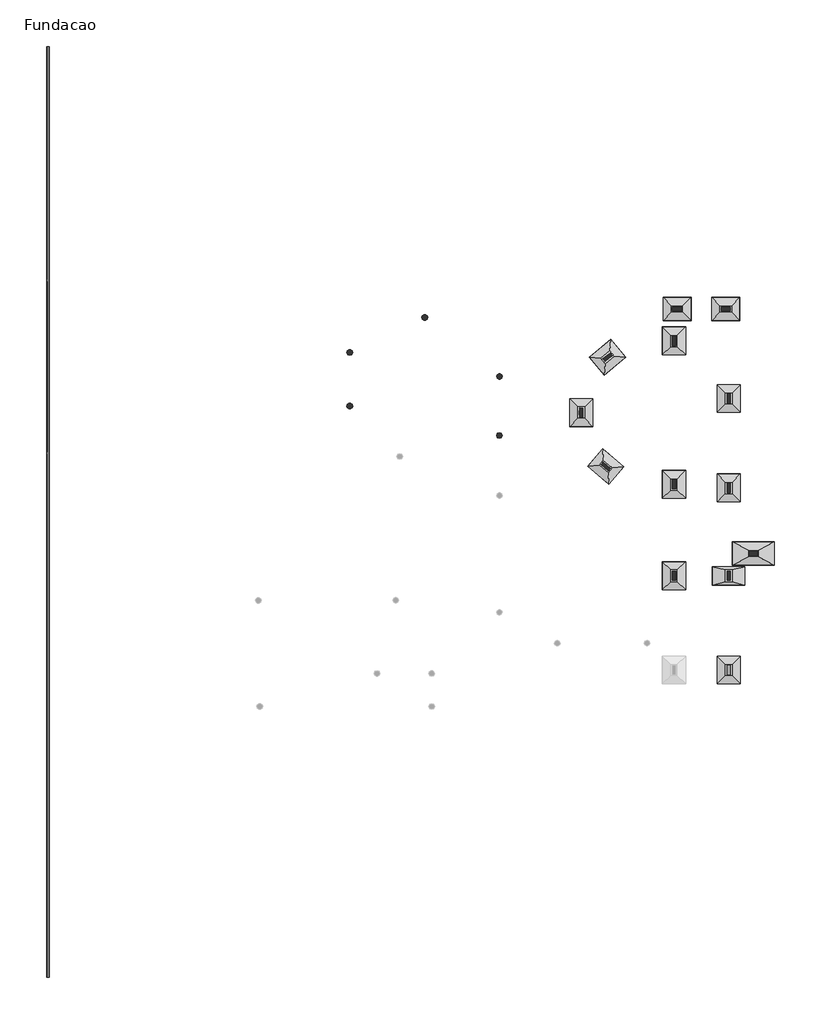
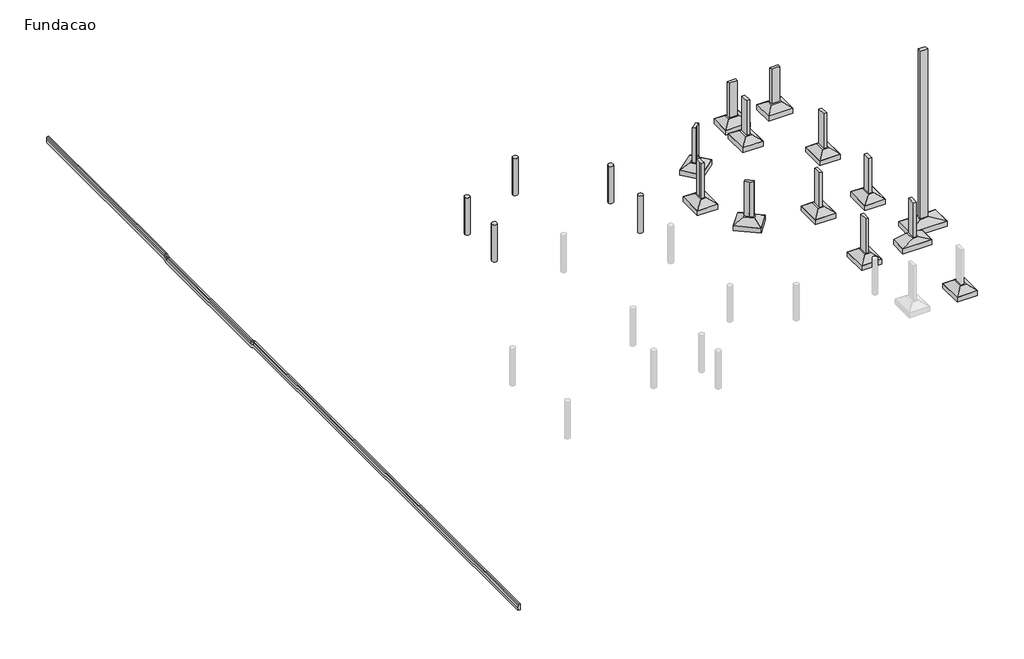
# One storey, part 2 of 2: 17 columns, 13 fasteners, 1 proxy.
"""IFC4 building model written with IfcOpenShell, lengths in millimetres."""

import ifcopenshell
import ifcopenshell.guid

model = None  # the IFC model being written
_history = None  # IfcOwnerHistory: only IFC2X3 demands one
_inside = {}  # id of a spatial element -> (the spatial element, [elements in it])
_under = {}  # id of a project, library or spatial element -> (it, [spatial elements below it])
_declared = {}  # id of a project -> (the project, [libraries it declares])
_typed = {}  # id of a type object -> (the type object, [elements of that type])
_made_of = {}  # id of a material, layer set ... -> (it, [elements and type objects made of it])


def new_model(schema):
    """Start an empty IFC model of exactly this schema.

    Asked for "IFC4X3", IfcOpenShell would pick the latest addendum, in which some entities
    have other attributes; the version numbers below select the first issue.
    IFC2X3 requires an IfcOwnerHistory on every rooted entity: one is made here for all.
    """
    global model, _history
    if schema == "IFC4X3":
        model = ifcopenshell.file(schema_version=(4, 3, 0, 0))
    else:
        model = ifcopenshell.file(schema=schema)
    _inside.clear()
    _under.clear()
    _declared.clear()
    _typed.clear()
    _made_of.clear()
    _history = None
    if model.schema == "IFC2X3":
        org = make("IfcOrganization", Name="unknown")
        user = make(
            "IfcPersonAndOrganization",
            ThePerson=make("IfcPerson", FamilyName="unknown"),
            TheOrganization=org,
        )
        app = make(
            "IfcApplication",
            ApplicationDeveloper=org,
            Version="unknown",
            ApplicationFullName="unknown",
            ApplicationIdentifier="unknown",
        )
        _history = make(
            "IfcOwnerHistory",
            OwningUser=user,
            OwningApplication=app,
            ChangeAction="ADDED",
            CreationDate=0,
        )
    return model


def make(cls, **values):
    """One entity of the class cls with the attributes given. An attribute that is None is left unset."""
    return model.create_entity(
        cls, **{name: value for name, value in values.items() if value is not None}
    )


def rooted(cls, **values):
    """An entity with a GlobalId (a new one), such as an element, a storey or a relation."""
    return make(cls, GlobalId=ifcopenshell.guid.new(), OwnerHistory=_history, **values)


def si_unit(unit_type, name, prefix=None):
    """IfcSIUnit, for example si_unit("LENGTHUNIT", "METRE", prefix="MILLI")."""
    return make("IfcSIUnit", UnitType=unit_type, Prefix=prefix, Name=name)


def assignment(units):
    """IfcUnitAssignment: the units of a project."""
    return None if units is None else make("IfcUnitAssignment", Units=units)


def point(xyz):
    """IfcCartesianPoint."""
    return None if xyz is None else make("IfcCartesianPoint", Coordinates=xyz)


def direction(xyz):
    """IfcDirection."""
    return None if xyz is None else make("IfcDirection", DirectionRatios=xyz)


def frame(location, z_axis=None, x_axis=None):
    """IfcAxis2Placement3D, a coordinate frame: its origin and axes. An axis left out is left unset."""
    return make(
        "IfcAxis2Placement3D",
        Location=point(location),
        Axis=direction(z_axis),
        RefDirection=direction(x_axis),
    )


def origin():
    """The frame at (0, 0, 0) with its axes left unset."""
    return frame((0.0, 0.0, 0.0))


def place(relative_to, where):
    """IfcLocalPlacement: puts the frame where relative to a parent placement (None: the world)."""
    return make(
        "IfcLocalPlacement", PlacementRelTo=relative_to, RelativePlacement=where
    )


def context(
    kind, dimensions, precision=None, world=None, true_north=None, identifier=None
):
    """IfcGeometricRepresentationContext, for example the 3D "Model" context."""
    return make(
        "IfcGeometricRepresentationContext",
        ContextIdentifier=identifier,
        ContextType=kind,
        CoordinateSpaceDimension=dimensions,
        Precision=precision,
        WorldCoordinateSystem=world,
        TrueNorth=true_north,
    )


def project(units=None, contexts=None):
    """IfcProject with its units and contexts."""
    return rooted(
        "IfcProject",
        Name="project",
        RepresentationContexts=contexts,
        UnitsInContext=assignment(units),
    )


def spatial(cls, under=None, at=None, **own):
    """A site, building, storey or space (cls), placed at a placement, below another one or the project."""
    s = rooted(cls, ObjectPlacement=at, **own)
    if under is not None:
        _under.setdefault(under.id(), (under, []))[1].append(s)
    return s


def polyline(points):
    """IfcPolyline through the points."""
    return make("IfcPolyline", Points=[point(p) for p in points])


def circle_curve(where, radius):
    """IfcCircle in the frame where."""
    return make("IfcCircle", Position=where, Radius=radius)


def ellipse_curve(where, semi_axis1, semi_axis2):
    """IfcEllipse in the frame where."""
    return make(
        "IfcEllipse", Position=where, SemiAxis1=semi_axis1, SemiAxis2=semi_axis2
    )


def outline(outer, holes=None, kind="AREA"):
    """IfcArbitraryClosedProfileDef: a profile drawn as a closed curve; with holes, ...WithVoids."""
    if holes is None:
        return make("IfcArbitraryClosedProfileDef", ProfileType=kind, OuterCurve=outer)
    return make(
        "IfcArbitraryProfileDefWithVoids",
        ProfileType=kind,
        OuterCurve=outer,
        InnerCurves=holes,
    )


def extrude(swept, where, along, depth):
    """IfcExtrudedAreaSolid: the profile swept, set in the frame where, extruded along a direction by depth."""
    return make(
        "IfcExtrudedAreaSolid",
        SweptArea=swept,
        Position=where,
        ExtrudedDirection=direction(along),
        Depth=depth,
    )


def faces_of(points, faces, orient=None, outer=None):
    """IfcFace entities. A face is a list of loops; a loop is a list of indices into points, from 0.

    orient and outer hold one flag for each loop. By default every Orientation is true, the
    first loop of a face is its IfcFaceOuterBound and the others are IfcFaceBound.
    """
    made = []
    for i, loops in enumerate(faces):
        bounds = []
        for j, loop in enumerate(loops):
            is_outer = j == 0 if outer is None else outer[i][j]
            bounds.append(
                make(
                    "IfcFaceOuterBound" if is_outer else "IfcFaceBound",
                    Bound=make("IfcPolyLoop", Polygon=[points[k] for k in loop]),
                    Orientation=True if orient is None else orient[i][j],
                )
            )
        made.append(make("IfcFace", Bounds=bounds))
    return made


def faceted_brep(points, faces, orient=None, outer=None, voids=None):
    """IfcFacetedBrep: a solid bounded by flat faces; with voids (closed shells), ...WithVoids."""
    shared = [point(p) for p in points]
    hull = make("IfcClosedShell", CfsFaces=faces_of(shared, faces, orient, outer))
    if voids is None:
        return make("IfcFacetedBrep", Outer=hull)
    return make(
        "IfcFacetedBrepWithVoids",
        Outer=hull,
        Voids=[
            make(cls, CfsFaces=faces_of(shared, fs, o, b)) for cls, fs, o, b in voids
        ],
    )


def shape(context_of_items, identifier, shape_type, items):
    """IfcShapeRepresentation: the items that make up one representation, for example the "Body"."""
    return make(
        "IfcShapeRepresentation",
        ContextOfItems=context_of_items,
        RepresentationIdentifier=identifier,
        RepresentationType=shape_type,
        Items=items,
    )


def source(mapping_origin, context_of_items, identifier, shape_type, items):
    """IfcRepresentationMap: a shape defined once, which mapped items show again and again."""
    return make(
        "IfcRepresentationMap",
        MappingOrigin=mapping_origin,
        MappedRepresentation=shape(context_of_items, identifier, shape_type, items),
    )


def transform(
    local_origin,
    x_axis=None,
    y_axis=None,
    z_axis=None,
    scale=None,
    scale2=None,
    scale3=None,
    uniform=True,
):
    """IfcCartesianTransformationOperator3D, or its non-uniform kind. x_axis, y_axis, z_axis: its Axis1, 2, 3."""
    if uniform:
        return make(
            "IfcCartesianTransformationOperator3D",
            Axis1=direction(x_axis),
            Axis2=direction(y_axis),
            LocalOrigin=point(local_origin),
            Scale=scale,
            Axis3=direction(z_axis),
        )
    return make(
        "IfcCartesianTransformationOperator3DnonUniform",
        Axis1=direction(x_axis),
        Axis2=direction(y_axis),
        LocalOrigin=point(local_origin),
        Scale=scale,
        Axis3=direction(z_axis),
        Scale2=scale2,
        Scale3=scale3,
    )


def mapped(mapping_source, mapping_target):
    """IfcMappedItem: shows the shape of a source again, moved by a transform."""
    return make(
        "IfcMappedItem", MappingSource=mapping_source, MappingTarget=mapping_target
    )


def made_of(thing, what):
    """Note that an element or type object is made of a material, layer set ...; save() writes the relation."""
    if what is not None:
        _made_of.setdefault(what.id(), (what, []))[1].append(thing)
    return thing


def element(
    cls,
    number,
    at=None,
    inside=None,
    cuts=None,
    type_object=None,
    material=None,
    context=None,
    identifier="Body",
    shape_type=None,
    held_by="IfcProductDefinitionShape",
    body=None,
    shapes=None,
    **own,
):
    """One element of the class cls, such as IfcWall. Its Tag is "e" and its number.

    at: its placement. inside: the storey or other place that contains it. cuts: it is an
    opening in that element (IfcRelVoidsElement). A single representation is given by context,
    identifier, shape_type and body (its items); several are given by shapes. held_by: the class
    of the entity that holds the representations. save() writes the other relations.
    """
    e = rooted(cls, Tag="e%d" % number, ObjectPlacement=at, **own)
    if body is not None:
        shapes = [shape(context, identifier, shape_type, body)]
    if shapes is not None:
        e.Representation = make(held_by, Representations=shapes)
    if inside is not None:
        _inside.setdefault(inside.id(), (inside, []))[1].append(e)
    if cuts is not None:
        rooted(
            "IfcRelVoidsElement", RelatingBuildingElement=cuts, RelatedOpeningElement=e
        )
    if type_object is not None:
        _typed.setdefault(type_object.id(), (type_object, []))[1].append(e)
    return made_of(e, material)


def aggregate(whole, parts):
    """IfcRelAggregates: a whole, such as a stair, and the parts it consists of."""
    return rooted("IfcRelAggregates", RelatingObject=whole, RelatedObjects=parts)


def save(model, path):
    """Write the relations noted so far, then the file.

    IfcRelAggregates (storeys below a building ...), IfcRelContainedInSpatialStructure (elements
    in a storey), IfcRelDefinesByType, IfcRelAssociatesMaterial and IfcRelDeclares: one each for
    every whole, place, type object, material and project.
    """
    for whole, parts in _under.values():
        aggregate(whole, parts)
    for where, things in _inside.values():
        rooted(
            "IfcRelContainedInSpatialStructure",
            RelatedElements=things,
            RelatingStructure=where,
        )
    for kind, things in _typed.values():
        rooted("IfcRelDefinesByType", RelatedObjects=things, RelatingType=kind)
    for what, things in _made_of.values():
        rooted("IfcRelAssociatesMaterial", RelatedObjects=things, RelatingMaterial=what)
    for by, libraries in _declared.values():
        rooted("IfcRelDeclares", RelatingContext=by, RelatedDefinitions=libraries)
    model.write(path)


def plane_surface(at):
    """IfcPlane: the flat surface through the origin of the frame at, square to its z axis."""
    return make("IfcPlane", Position=at)


def cylinder_surface(at, radius):
    """IfcCylindricalSurface: all points at the distance radius from the z axis of the frame at."""
    return make("IfcCylindricalSurface", Position=at, Radius=radius)


def advanced_brep(points, edges, surfaces, faces):
    """IfcAdvancedBrep: a solid bounded by faces that lie on surfaces and meet in shared edges.

    An edge is (start, end): straight between two places in points (the first is 0);
    or (start, end, curve); or (start, end, curve, False) where it runs against its curve.
    A face is (place in surfaces, loops), or (place, loops, False) where it looks against
    its surface's normal. A loop lists edges by number (the first is 1), with a minus sign
    where the edge is run from its end to its start. The first loop is the outer one.
    """
    corners = [point(p) for p in points]
    vertices = [make("IfcVertexPoint", VertexGeometry=c) for c in corners]
    made = []
    for start, end, *more in edges:
        made.append(
            make(
                "IfcEdgeCurve",
                EdgeStart=vertices[start],
                EdgeEnd=vertices[end],
                EdgeGeometry=more[0] if more else make("IfcPolyline", Points=[corners[start], corners[end]]),
                SameSense=more[1] if len(more) > 1 else True,
            )
        )
    hull = []
    for where, loops, *sense in faces:
        bounds = []
        for j, loop in enumerate(loops):
            ring = [make("IfcOrientedEdge", EdgeElement=made[abs(k) - 1], Orientation=k > 0) for k in loop]
            bounds.append(
                make(
                    "IfcFaceOuterBound" if j == 0 else "IfcFaceBound",
                    Bound=make("IfcEdgeLoop", EdgeList=ring),
                    Orientation=True,
                )
            )
        hull.append(make("IfcAdvancedFace", Bounds=bounds, FaceSurface=surfaces[where], SameSense=sense[0] if sense else True))
    return make("IfcAdvancedBrep", Outer=make("IfcClosedShell", CfsFaces=hull))


def meio_fio_meio_fio_c5939b1e(model_context):
    return source(origin(), model_context, "Body", "AdvancedBrep", [
        advanced_brep(
        [(-19460.281307, 17327.5225294, 100.0), (-19460.281307, 17327.5225294, -200.0), (-19580.281307, 17327.5225294, -200.0), (-19580.281307, 17327.5225294, -50.0), (-19560.334366, 17327.5225294, 74.7371665), (-19530.7107394, 17327.5225294, 100.0), (-19460.281307, 7304.4300153, 100.0), (-19460.281307, 7104.4300153, 20.0), (-19460.281307, 4.4300153, 20.0), (-19460.281307, -195.5699847, 100.0), (-19460.281307, -22700.938406, 100.0), (-19460.281307, -22700.938406, -200.0), (-19460.281307, -253.3447058, -200.0), (-19460.281307, -53.3447058, -280.0), (-19460.281307, 7162.2047364, -280.0), (-19460.281307, 7362.2047364, -200.0), (-19580.281307, 7362.2047364, -200.0), (-19580.281307, 7162.2047364, -280.0), (-19580.281307, -53.3447058, -280.0), (-19580.281307, -253.3447058, -200.0), (-19580.281307, -22700.938406, -200.0), (-19580.281307, -22700.938406, -50.0), (-19580.281307, -224.4573452, -50.0), (-19580.281307, -24.4573452, -130.0), (-19580.281307, 7133.3173758, -130.0), (-19580.281307, 7333.3173758, -50.0), (-19560.334366, 7309.2951925, 74.7371665), (-19530.7107394, 7304.4300153, 100.0), (-19560.334366, 7109.2951925, -5.2628335), (-19530.7107394, 7104.4300153, 20.0), (-19560.334366, -0.4351619, -5.2628335), (-19530.7107394, 4.4300153, 20.0), (-19560.334366, -200.4351619, 74.7371665), (-19530.7107394, -195.5699847, 100.0), (-19530.7107394, -22700.938406, 100.0), (-19560.334366, -22700.938406, 74.7371665)],
        [
            (0, 1),
            (1, 2),
            (2, 3),
            (3, 4),
            (4, 5, circle_curve(frame((-19530.7107394, 17327.5225294, 70.0), z_axis=(0.0, 1.0, 0.0), x_axis=(-1.0, 0.0, 0.0)), 30.0)),
            (5, 0),
            (0, 6),
            (6, 7),
            (7, 8),
            (8, 9),
            (9, 10),
            (10, 11),
            (11, 12),
            (12, 13),
            (13, 14),
            (14, 15),
            (15, 1),
            (15, 16),
            (16, 2),
            (16, 17),
            (17, 18),
            (18, 19),
            (19, 20),
            (20, 21),
            (21, 22),
            (22, 23),
            (23, 24),
            (24, 25),
            (25, 3),
            (25, 26),
            (26, 4),
            (26, 27, ellipse_curve(frame((-19530.7107394, 7310.2074874, 70.0), z_axis=(0.0, 0.9819563867314226, 0.18910752115494767), x_axis=(0.0, 0.18910752115494667, -0.9819563867314226)), 30.551255, 30.0)),
            (27, 5),
            (27, 6),
            (14, 17),
            (24, 28),
            (28, 26),
            (28, 29, ellipse_curve(frame((-19530.7107394, 7110.2074874, -10.0), z_axis=(0.0, 0.9819563867314226, 0.18910752115494764), x_axis=(0.0, -0.18910752115494842, 0.9819563867314223)), 30.551255, 30.0)),
            (29, 27),
            (29, 7),
            (13, 18),
            (23, 30),
            (30, 28),
            (30, 31, ellipse_curve(frame((-19530.7107394, -1.3474568, -10.0), z_axis=(0.0, 0.9819563867314217, -0.1891075211549513), x_axis=(0.0, 0.18910752115495252, 0.9819563867314217)), 30.551255, 30.0)),
            (31, 29),
            (31, 8),
            (12, 19),
            (22, 32),
            (32, 30),
            (32, 33, ellipse_curve(frame((-19530.7107394, -201.3474568, 70.0), z_axis=(0.0, 0.9819563867314217, -0.18910752115495139), x_axis=(0.0, -0.18910752115495078, -0.9819563867314218)), 30.551255, 30.0)),
            (33, 31),
            (33, 9),
            (10, 34),
            (34, 35, circle_curve(frame((-19530.7107394, -22700.938406, 70.0), z_axis=(0.0, -1.0, 0.0), x_axis=(-1.0, 0.0, 0.0)), 30.0)),
            (35, 21),
            (20, 11),
            (35, 32),
            (34, 33),
        ],
        [
            plane_surface(frame((-19460.281307, 17327.5225294, 100.0), z_axis=(0.0, 1.0, 0.0), x_axis=(0.0, 0.0, 1.0))),
            plane_surface(frame((-19460.281307, 17327.5225294, 100.0), z_axis=(1.0, 0.0, 0.0), x_axis=(0.0, -1.0, 0.0))),
            plane_surface(frame((-19460.281307, 17327.5225294, -200.0), z_axis=(0.0, 0.0, -1.0), x_axis=(0.0, -1.0, 0.0))),
            plane_surface(frame((-19580.281307, 17327.5225294, -200.0), z_axis=(-1.0, 0.0, 0.0), x_axis=(0.0, -1.0, 0.0))),
            plane_surface(frame((-19580.281307, 17327.5225294, -50.0), z_axis=(-0.9874542202157147, 0.0, 0.15790555081495689), x_axis=(0.0, -1.0, 0.0))),
            cylinder_surface(frame((-19530.7107394, 17327.5225294, 70.0), z_axis=(0.0, 1.0, 0.0), x_axis=(-1.0, 0.0, 0.0)), 30.0),
            plane_surface(frame((-19530.7107394, 17327.5225294, 100.0), z_axis=(0.0, 0.0, 1.0), x_axis=(0.0, -1.0, 0.0))),
            plane_surface(frame((-19460.281307, 7362.2047364, -200.0), z_axis=(0.0, 0.3713906763540969, -0.9284766908852621), x_axis=(0.0, -0.9284766908852621, -0.3713906763540969))),
            plane_surface(frame((-19580.281307, 7333.3173758, -50.0), z_axis=(-0.9874542202157147, -0.05864464931723302, 0.1466116232930858), x_axis=(0.0, -0.9284766908852622, -0.3713906763540966))),
            cylinder_surface(frame((-19530.7107394, 7315.5717356, 72.1456993), z_axis=(0.0, 0.9284766908852621, 0.3713906763540969), x_axis=(-1.0, 0.0, 0.0)), 30.0),
            plane_surface(frame((-19530.7107394, 7304.4300153, 100.0), z_axis=(0.0, -0.37139067635409667, 0.9284766908852622), x_axis=(0.0, -0.9284766908852622, -0.37139067635409667))),
            plane_surface(frame((-19460.281307, 7162.2047364, -280.0), z_axis=(0.0, 0.0, -1.0), x_axis=(0.0, -1.0, 0.0))),
            plane_surface(frame((-19580.281307, 7133.3173758, -130.0), z_axis=(-0.9874542202157146, 0.0, 0.15790555081495686), x_axis=(0.0, -1.0, 0.0))),
            cylinder_surface(frame((-19530.7107394, 7104.4300153, -10.0), z_axis=(0.0, 1.0, 0.0), x_axis=(-1.0, 0.0, 0.0)), 30.0),
            plane_surface(frame((-19530.7107394, 7104.4300153, 20.0), z_axis=(0.0, 0.0, 1.0), x_axis=(0.0, -1.0, 0.0))),
            plane_surface(frame((-19460.281307, -53.3447058, -280.0), z_axis=(0.0, -0.37139067635410367, -0.9284766908852594), x_axis=(0.0, -0.9284766908852594, 0.37139067635410367))),
            plane_surface(frame((-19580.281307, -24.4573452, -130.0), z_axis=(-0.9874542202157147, 0.05864464931723411, 0.14661162329308536), x_axis=(0.0, -0.9284766908852594, 0.37139067635410355))),
            cylinder_surface(frame((-19530.7107394, -6.711705, -7.8543007), z_axis=(0.0, 0.9284766908852593, -0.3713906763541038), x_axis=(-1.0, 0.0, 0.0)), 30.0),
            plane_surface(frame((-19530.7107394, 4.4300153, 20.0), z_axis=(0.0, 0.3713906763541038, 0.9284766908852593), x_axis=(0.0, -0.9284766908852593, 0.3713906763541038))),
            plane_surface(frame((-19460.281307, -22700.938406, 100.0), z_axis=(0.0, -1.0, 0.0), x_axis=(0.0, 0.0, 1.0))),
            plane_surface(frame((-19460.281307, -253.3447058, -200.0), z_axis=(0.0, 0.0, -1.0), x_axis=(0.0, -1.0, 0.0))),
            plane_surface(frame((-19580.281307, -224.4573452, -50.0), z_axis=(-0.9874542202157146, 0.0, 0.15790555081495683), x_axis=(0.0, -1.0, 0.0))),
            cylinder_surface(frame((-19530.7107394, -195.5699847, 70.0), z_axis=(0.0, 1.0, 0.0), x_axis=(-1.0, 0.0, 0.0)), 30.0),
            plane_surface(frame((-19530.7107394, -195.5699847, 100.0), z_axis=(0.0, 0.0, 1.0), x_axis=(0.0, -1.0, 0.0))),
        ],
        [
            (0, [[1, 2, 3, 4, 5, 6]]),
            (1, [[-1, 7, 8, 9, 10, 11, 12, 13, 14, 15, 16, 17]]),
            (2, [[-2, -17, 18, 19]]),
            (3, [[-3, -19, 20, 21, 22, 23, 24, 25, 26, 27, 28, 29]]),
            (4, [[-4, -29, 30, 31]]),
            (5, [[-5, -31, 32, 33]]),
            (6, [[-6, -33, 34, -7]]),
            (7, [[-18, -16, 35, -20]]),
            (8, [[-30, -28, 36, 37]]),
            (9, [[-32, -37, 38, 39]]),
            (10, [[-34, -39, 40, -8]]),
            (11, [[-35, -15, 41, -21]]),
            (12, [[-36, -27, 42, 43]]),
            (13, [[-38, -43, 44, 45]]),
            (14, [[-40, -45, 46, -9]]),
            (15, [[-41, -14, 47, -22]]),
            (16, [[-42, -26, 48, 49]]),
            (17, [[-44, -49, 50, 51]]),
            (18, [[-46, -51, 52, -10]]),
            (19, [[53, 54, 55, -24, 56, -12]]),
            (20, [[-47, -13, -56, -23]]),
            (21, [[-48, -25, -55, 57]]),
            (22, [[-50, -57, -54, 58]]),
            (23, [[-52, -58, -53, -11]]),
        ],
    ),
    ])


def s14_8166d2be(model_context):
    return source(origin(), model_context, "Body", "SolidModel", [
        faceted_brep([(-55.0, 0.0, 0.0), (-345.0, 0.0, 0.0), (-345.0, -400.0, 0.0), (-55.0, -400.0, 0.0), (300.0, 700.0, -250.0), (300.0, -1100.0, -250.0), (-700.0, -1100.0, -250.0), (-700.0, 700.0, -250.0)], [[[0, 1, 2, 3]], [[4, 5, 6, 7]], [[4, 7, 1, 0]], [[7, 6, 2, 1]], [[6, 5, 3, 2]], [[5, 4, 0, 3]]]),
        extrude(outline(polyline([(300.0, 700.0), (300.0, -1100.0), (-700.0, -1100.0), (-700.0, 700.0), (300.0, 700.0)])), frame((0.0, 0.0, -500.0), z_axis=(0.0, 0.0, 1.0), x_axis=(1.0, 0.0, 0.0)), (0.0, 0.0, 1.0), 250.0),
    ])


def sps1_6b3be553(model_context):
    return source(origin(), model_context, "Body", "SolidModel", [
        faceted_brep([(-55.0, 50.0, 0.0), (-345.0, 50.0, 0.0), (-345.0, -450.0, 0.0), (-55.0, -450.0, 0.0), (300.0, 400.0, -250.0), (300.0, -800.0, -250.0), (-700.0, -800.0, -250.0), (-700.0, 400.0, -250.0)], [[[0, 1, 2, 3]], [[4, 5, 6, 7]], [[4, 7, 1, 0]], [[7, 6, 2, 1]], [[6, 5, 3, 2]], [[5, 4, 0, 3]]]),
        extrude(outline(polyline([(300.0, 400.0), (300.0, -800.0), (-700.0, -800.0), (-700.0, 400.0), (300.0, 400.0)])), frame((0.0, 0.0, -500.0), z_axis=(0.0, 0.0, 1.0), x_axis=(1.0, 0.0, 0.0)), (0.0, 0.0, 1.0), 250.0),
    ])


def sps11_3ae28187(model_context):
    return source(origin(), model_context, "Body", "SolidModel", [
        faceted_brep([(-55.0, 50.0, 0.0), (-345.0, 50.0, 0.0), (-345.0, -450.0, 0.0), (-55.0, -450.0, 0.0), (500.0, 200.0, -250.0), (500.0, -600.0, -250.0), (-900.0, -600.0, -250.0), (-900.0, 200.0, -250.0)], [[[0, 1, 2, 3]], [[4, 5, 6, 7]], [[4, 7, 1, 0]], [[7, 6, 2, 1]], [[6, 5, 3, 2]], [[5, 4, 0, 3]]]),
        extrude(outline(polyline([(500.0, 200.0), (500.0, -600.0), (-900.0, -600.0), (-900.0, 200.0), (500.0, 200.0)])), frame((0.0, 0.0, -500.0), z_axis=(0.0, 0.0, 1.0), x_axis=(1.0, 0.0, 0.0)), (0.0, 0.0, 1.0), 250.0),
    ])


model = new_model("IFC4")

# Units and contexts
model_context = context("Model", 3, world=origin())
ifc_project = project(units=[si_unit("LENGTHUNIT", "METRE", prefix="MILLI")], contexts=[model_context])

# Site, building, storey
site = spatial("IfcSite", under=ifc_project)
building = spatial("IfcBuilding", under=site)
storey = spatial("IfcBuildingStorey", under=building, Name="Fundacao", Elevation=-1200.0)

# Proxy
placement = place(None, origin())
meio_fio_meio_fio_shape = meio_fio_meio_fio_c5939b1e(model_context)
element("IfcBuildingElementProxy", 1, Name="MEIO-FIO : MEIO-FIO", ObjectType="MEIO-FIO : MEIO-FIO", at=placement, inside=storey, context=model_context, shape_type="MappedRepresentation", body=[
    mapped(meio_fio_meio_fio_shape, transform((0.0, 0.0, 0.0), x_axis=(1.0, 0.0, 0.0), y_axis=(0.0, 1.0, 0.0), z_axis=(0.0, 0.0, 1.0))),
])

# Columns
element("IfcColumn", 2, ObjectType="TQS - Pilar circular : TQS - Pilar circular 25.0cm", at=placement, inside=storey, context=model_context, shape_type="AdvancedBrep", body=[
    advanced_brep(
    [(-3446.281307, 5679.4300153, -1500.0), (-3196.281307, 5679.4300153, -1500.0), (-3446.281307, 5679.4300153, 430.0), (-3402.499945, 5774.4486073, 430.0), (-3240.0409229, 5774.4300153, 430.0), (-3196.281307, 5679.4300153, 430.0), (-3240.0409229, 5584.4300153, 430.0), (-3402.499945, 5584.4114233, 430.0)],
    [
        (0, 1, circle_curve(frame((-3321.281307, 5679.4300153, -1500.0), z_axis=(0.0, 0.0, -1.0), x_axis=(1.0, 0.0, 0.0)), 125.0)),
        (1, 0, circle_curve(frame((-3321.281307, 5679.4300153, -1500.0), z_axis=(0.0, 0.0, -1.0), x_axis=(1.0, 0.0, 0.0)), 125.0)),
        (2, 3, circle_curve(frame((-3321.281307, 5679.4300153, 430.0), z_axis=(0.0, 0.0, -1.0), x_axis=(1.0, 0.0, 0.0)), 125.0)),
        (3, 4, circle_curve(frame((-3321.281307, 5679.4300153, 430.0), z_axis=(0.0, 0.0, -1.0), x_axis=(1.0, 0.0, 0.0)), 125.0)),
        (4, 5, circle_curve(frame((-3321.281307, 5679.4300153, 430.0), z_axis=(0.0, 0.0, -1.0), x_axis=(1.0, 0.0, 0.0)), 125.0)),
        (5, 1),
        (0, 2),
        (5, 6, circle_curve(frame((-3321.281307, 5679.4300153, 430.0), z_axis=(0.0, 0.0, -1.0), x_axis=(1.0, 0.0, 0.0)), 125.0)),
        (6, 7, circle_curve(frame((-3321.281307, 5679.4300153, 430.0), z_axis=(0.0, 0.0, -1.0), x_axis=(1.0, 0.0, 0.0)), 125.0)),
        (7, 2, circle_curve(frame((-3321.281307, 5679.4300153, 430.0), z_axis=(0.0, 0.0, -1.0), x_axis=(1.0, 0.0, 0.0)), 125.0)),
    ],
    [
        plane_surface(frame((-3196.281307, 5679.4300153, -1500.0), z_axis=(0.0, 0.0, -1.0), x_axis=(0.0, -1.0, 0.0))),
        cylinder_surface(frame((-3321.281307, 5679.4300153, -1500.0), z_axis=(0.0, 0.0, 1.0), x_axis=(1.0, 0.0, 0.0)), 125.0),
        plane_surface(frame((-3196.281307, 5679.4300153, 430.0), z_axis=(0.0, 0.0, 1.0), x_axis=(0.0, 1.0, 0.0))),
    ],
    [
        (0, [[1, 2]]),
        (1, [[3, 4, 5, 6, -1, 7]]),
        (1, [[8, 9, 10, -7, -2, -6]]),
        (2, [[-10, -9, -8, -5, -4, -3]]),
    ],
),
])
element("IfcColumn", 3, ObjectType="TQS - Pilar circular : TQS - Pilar circular 25.0cm", at=placement, inside=storey, context=model_context, shape_type="AdvancedBrep", body=[
    advanced_brep(
    [(-232.281307, 604.4300152, -1500.0), (17.718693, 604.4300152, -1500.0), (-232.281307, 604.4300152, 430.0), (-202.281307, 685.6703993, 430.0), (-12.281307, 685.6703993, 430.0), (17.718693, 604.4300152, 430.0), (-12.281307, 523.1896312, 430.0), (-202.281307, 523.1896312, 430.0)],
    [
        (0, 1, circle_curve(frame((-107.281307, 604.4300152, -1500.0), z_axis=(0.0, 0.0, -1.0), x_axis=(1.0, 0.0, 0.0)), 125.0)),
        (1, 0, circle_curve(frame((-107.281307, 604.4300152, -1500.0), z_axis=(0.0, 0.0, -1.0), x_axis=(1.0, 0.0, 0.0)), 125.0)),
        (2, 3, circle_curve(frame((-107.281307, 604.4300152, 430.0), z_axis=(0.0, 0.0, -1.0), x_axis=(1.0, 0.0, 0.0)), 125.0)),
        (3, 4, circle_curve(frame((-107.281307, 604.4300152, 430.0), z_axis=(0.0, 0.0, -1.0), x_axis=(1.0, 0.0, 0.0)), 125.0)),
        (4, 5, circle_curve(frame((-107.281307, 604.4300152, 430.0), z_axis=(0.0, 0.0, -1.0), x_axis=(1.0, 0.0, 0.0)), 125.0)),
        (5, 1),
        (0, 2),
        (5, 6, circle_curve(frame((-107.281307, 604.4300152, 430.0), z_axis=(0.0, 0.0, -1.0), x_axis=(1.0, 0.0, 0.0)), 125.0)),
        (6, 7, circle_curve(frame((-107.281307, 604.4300152, 430.0), z_axis=(0.0, 0.0, -1.0), x_axis=(1.0, 0.0, 0.0)), 125.0)),
        (7, 2, circle_curve(frame((-107.281307, 604.4300152, 430.0), z_axis=(0.0, 0.0, -1.0), x_axis=(1.0, 0.0, 0.0)), 125.0)),
    ],
    [
        plane_surface(frame((17.718693, 604.4300152, -1500.0), z_axis=(0.0, 0.0, -1.0), x_axis=(0.0, -1.0, 0.0))),
        cylinder_surface(frame((-107.281307, 604.4300152, -1500.0), z_axis=(0.0, 0.0, 1.0), x_axis=(1.0, 0.0, 0.0)), 125.0),
        plane_surface(frame((17.718693, 604.4300152, 430.0), z_axis=(0.0, 0.0, 1.0), x_axis=(0.0, 1.0, 0.0))),
    ],
    [
        (0, [[1, 2]]),
        (1, [[3, 4, 5, 6, -1, 7]]),
        (1, [[8, 9, 10, -7, -2, -6]]),
        (2, [[-10, -9, -8, -5, -4, -3]]),
    ],
),
])
element("IfcColumn", 4, ObjectType="TQS - Pilar circular : TQS - Pilar circular 25.0cm", at=placement, inside=storey, context=model_context, shape_type="AdvancedBrep", body=[
    advanced_brep(
    [(-232.281307, 3141.9300152, -1500.0), (17.718693, 3141.9300152, -1500.0), (-232.281307, 3141.9300152, 430.0), (-202.281307, 3223.1703993, 430.0), (-12.281307, 3223.1703993, 430.0), (17.718693, 3141.9300152, 430.0), (-12.281307, 3060.6896312, 430.0), (-202.281307, 3060.6896312, 430.0)],
    [
        (0, 1, circle_curve(frame((-107.281307, 3141.9300152, -1500.0), z_axis=(0.0, 0.0, -1.0), x_axis=(1.0, 0.0, 0.0)), 125.0)),
        (1, 0, circle_curve(frame((-107.281307, 3141.9300152, -1500.0), z_axis=(0.0, 0.0, -1.0), x_axis=(1.0, 0.0, 0.0)), 125.0)),
        (2, 3, circle_curve(frame((-107.281307, 3141.9300152, 430.0), z_axis=(0.0, 0.0, -1.0), x_axis=(1.0, 0.0, 0.0)), 125.0)),
        (3, 4, circle_curve(frame((-107.281307, 3141.9300152, 430.0), z_axis=(0.0, 0.0, -1.0), x_axis=(1.0, 0.0, 0.0)), 125.0)),
        (4, 5, circle_curve(frame((-107.281307, 3141.9300152, 430.0), z_axis=(0.0, 0.0, -1.0), x_axis=(1.0, 0.0, 0.0)), 125.0)),
        (5, 1),
        (0, 2),
        (5, 6, circle_curve(frame((-107.281307, 3141.9300152, 430.0), z_axis=(0.0, 0.0, -1.0), x_axis=(1.0, 0.0, 0.0)), 125.0)),
        (6, 7, circle_curve(frame((-107.281307, 3141.9300152, 430.0), z_axis=(0.0, 0.0, -1.0), x_axis=(1.0, 0.0, 0.0)), 125.0)),
        (7, 2, circle_curve(frame((-107.281307, 3141.9300152, 430.0), z_axis=(0.0, 0.0, -1.0), x_axis=(1.0, 0.0, 0.0)), 125.0)),
    ],
    [
        plane_surface(frame((17.718693, 3141.9300152, -1500.0), z_axis=(0.0, 0.0, -1.0), x_axis=(0.0, -1.0, 0.0))),
        cylinder_surface(frame((-107.281307, 3141.9300152, -1500.0), z_axis=(0.0, 0.0, 1.0), x_axis=(1.0, 0.0, 0.0)), 125.0),
        plane_surface(frame((17.718693, 3141.9300152, 430.0), z_axis=(0.0, 0.0, 1.0), x_axis=(0.0, 1.0, 0.0))),
    ],
    [
        (0, [[1, 2]]),
        (1, [[3, 4, 5, 6, -1, 7]]),
        (1, [[8, 9, 10, -7, -2, -6]]),
        (2, [[-10, -9, -8, -5, -4, -3]]),
    ],
),
])
element("IfcColumn", 5, ObjectType="TQS - Pilar circular : TQS - Pilar circular 25.0cm", at=placement, inside=storey, context=model_context, shape_type="AdvancedBrep", body=[
    advanced_brep(
    [(-6671.281307, 4171.2050153, -1500.0), (-6421.281307, 4171.2050153, -1500.0), (-6671.281307, 4171.2050153, 430.0), (-6630.281307, 4263.7739086, 430.0), (-6440.281307, 4237.4545436, 430.0), (-6421.281307, 4171.2050153, 430.0), (-6440.281307, 4104.955487, 430.0), (-6630.281307, 4078.636122, 430.0)],
    [
        (0, 1, circle_curve(frame((-6546.281307, 4171.2050153, -1500.0), z_axis=(0.0, 0.0, -1.0), x_axis=(1.0, 0.0, 0.0)), 125.0)),
        (1, 0, circle_curve(frame((-6546.281307, 4171.2050153, -1500.0), z_axis=(0.0, 0.0, -1.0), x_axis=(1.0, 0.0, 0.0)), 125.0)),
        (2, 3, circle_curve(frame((-6546.281307, 4171.2050153, 430.0), z_axis=(0.0, 0.0, -1.0), x_axis=(1.0, 0.0, 0.0)), 125.0)),
        (3, 4, circle_curve(frame((-6546.281307, 4171.2050153, 430.0), z_axis=(0.0, 0.0, -1.0), x_axis=(1.0, 0.0, 0.0)), 125.0)),
        (4, 5, circle_curve(frame((-6546.281307, 4171.2050153, 430.0), z_axis=(0.0, 0.0, -1.0), x_axis=(1.0, 0.0, 0.0)), 125.0)),
        (5, 1),
        (0, 2),
        (5, 6, circle_curve(frame((-6546.281307, 4171.2050153, 430.0), z_axis=(0.0, 0.0, -1.0), x_axis=(1.0, 0.0, 0.0)), 125.0)),
        (6, 7, circle_curve(frame((-6546.281307, 4171.2050153, 430.0), z_axis=(0.0, 0.0, -1.0), x_axis=(1.0, 0.0, 0.0)), 125.0)),
        (7, 2, circle_curve(frame((-6546.281307, 4171.2050153, 430.0), z_axis=(0.0, 0.0, -1.0), x_axis=(1.0, 0.0, 0.0)), 125.0)),
    ],
    [
        plane_surface(frame((-6421.281307, 4171.2050153, -1500.0), z_axis=(0.0, 0.0, -1.0), x_axis=(0.0, -1.0, 0.0))),
        cylinder_surface(frame((-6546.281307, 4171.2050153, -1500.0), z_axis=(0.0, 0.0, 1.0), x_axis=(1.0, 0.0, 0.0)), 125.0),
        plane_surface(frame((-6421.281307, 4171.2050153, 430.0), z_axis=(0.0, 0.0, 1.0), x_axis=(0.0, 1.0, 0.0))),
    ],
    [
        (0, [[1, 2]]),
        (1, [[3, 4, 5, 6, -1, 7]]),
        (1, [[8, 9, 10, -7, -2, -6]]),
        (2, [[-10, -9, -8, -5, -4, -3]]),
    ],
),
])
element("IfcColumn", 6, ObjectType="TQS - Pilar circular : TQS - Pilar circular 25.0cm", at=placement, inside=storey, context=model_context, shape_type="AdvancedBrep", body=[
    advanced_brep(
    [(-6666.2813069, 1866.7050153, -1500.0), (-6416.2813069, 1866.7050153, -1500.0), (-6666.2813069, 1866.7050153, 430.0), (-6630.281307, 1954.4774483, 430.0), (-6440.281307, 1940.3528259, 430.0), (-6416.2813069, 1866.7050153, 430.0), (-6440.281307, 1793.0572047, 430.0), (-6630.281307, 1778.9325823, 430.0)],
    [
        (0, 1, circle_curve(frame((-6541.2813069, 1866.7050153, -1500.0), z_axis=(0.0, 0.0, -1.0), x_axis=(1.0, 0.0, 0.0)), 125.0)),
        (1, 0, circle_curve(frame((-6541.2813069, 1866.7050153, -1500.0), z_axis=(0.0, 0.0, -1.0), x_axis=(1.0, 0.0, 0.0)), 125.0)),
        (2, 3, circle_curve(frame((-6541.2813069, 1866.7050153, 430.0), z_axis=(0.0, 0.0, -1.0), x_axis=(1.0, 0.0, 0.0)), 125.0)),
        (3, 4, circle_curve(frame((-6541.2813069, 1866.7050153, 430.0), z_axis=(0.0, 0.0, -1.0), x_axis=(1.0, 0.0, 0.0)), 125.0)),
        (4, 5, circle_curve(frame((-6541.2813069, 1866.7050153, 430.0), z_axis=(0.0, 0.0, -1.0), x_axis=(1.0, 0.0, 0.0)), 125.0)),
        (5, 1),
        (0, 2),
        (5, 6, circle_curve(frame((-6541.2813069, 1866.7050153, 430.0), z_axis=(0.0, 0.0, -1.0), x_axis=(1.0, 0.0, 0.0)), 125.0)),
        (6, 7, circle_curve(frame((-6541.2813069, 1866.7050153, 430.0), z_axis=(0.0, 0.0, -1.0), x_axis=(1.0, 0.0, 0.0)), 125.0)),
        (7, 2, circle_curve(frame((-6541.2813069, 1866.7050153, 430.0), z_axis=(0.0, 0.0, -1.0), x_axis=(1.0, 0.0, 0.0)), 125.0)),
    ],
    [
        plane_surface(frame((-6416.2813069, 1866.7050153, -1500.0), z_axis=(0.0, 0.0, -1.0), x_axis=(0.0, -1.0, 0.0))),
        cylinder_surface(frame((-6541.2813069, 1866.7050153, -1500.0), z_axis=(0.0, 0.0, 1.0), x_axis=(1.0, 0.0, 0.0)), 125.0),
        plane_surface(frame((-6416.2813069, 1866.7050153, 430.0), z_axis=(0.0, 0.0, 1.0), x_axis=(0.0, 1.0, 0.0))),
    ],
    [
        (0, [[1, 2]]),
        (1, [[3, 4, 5, 6, -1, 7]]),
        (1, [[8, 9, 10, -7, -2, -6]]),
        (2, [[-10, -9, -8, -5, -4, -3]]),
    ],
),
])
element("IfcColumn", 7, ObjectType="TQS - Pilar retangular : 14.0 x 40.0", at=placement, inside=storey, context=model_context, shape_type="Brep", body=[
    faceted_brep([(9822.718693, 5969.4300153, -1450.0), (9682.718693, 5969.4300153, -1450.0), (9422.718693, 5969.4300153, -1450.0), (9422.718693, 6109.4300153, -1450.0), (9822.718693, 6109.4300153, -1450.0), (9822.718693, 5969.4300153, 350.0), (9682.718693, 5969.4300153, 350.0), (9422.718693, 5969.4300153, 350.0), (9422.718693, 6109.4300153, 350.0), (9822.718693, 6109.4300153, 350.0)], [[[0, 1, 2, 3, 4]], [[5, 6, 7, 2, 1, 0]], [[7, 8, 3, 2]], [[8, 9, 4, 3]], [[9, 5, 0, 4]], [[5, 9, 8, 7, 6]]]),
])
element("IfcColumn", 8, ObjectType="TQS - Pilar retangular : 14.0 x 40.0", at=placement, inside=storey, context=model_context, shape_type="Brep", body=[
    faceted_brep([(7734.718693, 5969.4300153, -1450.0), (7474.7218272, 5969.4300153, -1450.0), (7334.718693, 5969.4300153, -1450.0), (7334.718693, 6109.4300153, -1450.0), (7734.718693, 6109.4300153, -1450.0), (7734.718693, 5969.4300153, 350.0), (7474.7218272, 5969.4300153, 350.0), (7334.718693, 5969.4300153, 350.0), (7334.718693, 6109.4300153, 350.0), (7734.718693, 6109.4300153, 350.0)], [[[0, 1, 2, 3, 4]], [[5, 6, 7, 2, 1, 0]], [[7, 8, 3, 2]], [[8, 9, 4, 3]], [[9, 5, 0, 4]], [[5, 9, 8, 7, 6]]]),
])
element("IfcColumn", 9, ObjectType="TQS - Pilar retangular : 14.0 x 40.0", at=placement, inside=storey, context=model_context, shape_type="Brep", body=[
    faceted_brep([(7334.7218272, 4470.7003679, -1450.0), (7334.7218272, 4614.8968948, -1450.0), (7334.7218272, 4870.7003679, -1450.0), (7474.7218272, 4870.7003679, -1450.0), (7474.7218272, 4470.7003679, -1450.0), (7334.7218272, 4470.7003679, -1250.0), (7334.7218272, 4470.7003679, 350.0), (7334.7218272, 4614.8968948, 350.0), (7334.7218272, 4870.7003679, 350.0), (7474.7218272, 4870.7003679, 350.0), (7474.7218272, 4870.7003679, -1250.0), (7474.7218272, 4470.7003679, 350.0), (7474.7218272, 4470.7003679, -1250.0)], [[[0, 1, 2, 3, 4]], [[2, 1, 0, 5, 6, 7, 8]], [[3, 2, 8, 9, 10]], [[4, 3, 10, 9, 11, 12]], [[0, 4, 12, 11, 6, 5]], [[8, 7, 6, 11, 9]]]),
])
element("IfcColumn", 10, ObjectType="TQS - Pilar retangular : 14.0 x 40.0", at=placement, inside=storey, context=model_context, shape_type="Brep", body=[
    faceted_brep([(7334.718693, -1696.0936198, -1450.0), (7334.718693, -1440.2725066, -1450.0), (7334.718693, -1296.0936198, -1450.0), (7474.718693, -1296.0936198, -1450.0), (7474.718693, -1696.0936198, -1450.0), (7334.718693, -1696.0936198, 350.0), (7334.718693, -1440.2725066, 350.0), (7334.718693, -1296.0936198, 350.0), (7334.718693, -1296.0936198, -1250.0), (7474.718693, -1296.0936198, 350.0), (7474.718693, -1296.0936198, -1250.0), (7474.718693, -1696.0936198, 350.0), (7474.718693, -1696.0936198, -1250.0)], [[[0, 1, 2, 3, 4]], [[2, 1, 0, 5, 6, 7, 8]], [[3, 2, 8, 7, 9, 10]], [[4, 3, 10, 9, 11, 12]], [[0, 4, 12, 11, 5]], [[7, 6, 5, 11, 9]]]),
])
element("IfcColumn", 11, ObjectType="TQS - Pilar retangular : 14.0 x 40.0", at=placement, inside=storey, context=model_context, shape_type="Brep", body=[
    faceted_brep([(7334.718693, -5630.1494451, -1450.0), (7334.718693, -5230.1494451, -1450.0), (7474.718693, -5230.1494451, -1450.0), (7474.718693, -5630.1494451, -1450.0), (7334.718693, -5630.1494451, 350.0), (7334.718693, -5230.1494451, 350.0), (7474.718693, -5230.1494451, 350.0), (7474.718693, -5230.1494451, -1250.0), (7474.718693, -5630.1494451, 350.0), (7474.718693, -5630.1494451, -1250.0)], [[[0, 1, 2, 3]], [[1, 0, 4, 5]], [[2, 1, 5, 6, 7]], [[3, 2, 7, 6, 8, 9]], [[0, 3, 9, 8, 4]], [[5, 4, 8, 6]]]),
])
element("IfcColumn", 12, ObjectType="TQS - Pilar retangular : 14.0 x 40.0", at=placement, inside=storey, context=model_context, shape_type="SweptSolid", body=[
    extrude(outline(polyline([(9682.718693, -5630.1494451), (9682.718693, -5230.1494451), (9822.718693, -5230.1494451), (9822.718693, -5630.1494451), (9682.718693, -5630.1494451)])), frame((0.0, 0.0, -1450.0), z_axis=(0.0, 0.0, 1.0), x_axis=(1.0, 0.0, 0.0)), (0.0, 0.0, 1.0), 1800.0),
])
element("IfcColumn", 13, ObjectType="TQS - Pilar retangular : 14.0 x 40.0", at=placement, inside=storey, context=model_context, shape_type="SweptSolid", body=[
    extrude(outline(polyline([(9682.718693, -1851.4011146), (9682.718693, -1451.4011146), (9822.718693, -1451.4011146), (9822.718693, -1851.4011146), (9682.718693, -1851.4011146)])), frame((0.0, 0.0, -1450.0), z_axis=(0.0, 0.0, 1.0), x_axis=(1.0, 0.0, 0.0)), (0.0, 0.0, 1.0), 1800.0),
])
element("IfcColumn", 14, ObjectType="TQS - Pilar retangular : 14.0 x 40.0", at=placement, inside=storey, context=model_context, shape_type="SweptSolid", body=[
    extrude(outline(polyline([(9682.718693, 1994.0144504), (9682.718693, 2394.0144504), (9822.718693, 2394.0144504), (9822.718693, 1994.0144504), (9682.718693, 1994.0144504)])), frame((0.0, 0.0, -1450.0), z_axis=(0.0, 0.0, 1.0), x_axis=(1.0, 0.0, 0.0)), (0.0, 0.0, 1.0), 1800.0),
])
element("IfcColumn", 15, ObjectType="TQS - Pilar retangular : 19.0 x 35.0", at=placement, inside=storey, context=model_context, shape_type="Brep", body=[
    faceted_brep([(10637.718693, -4375.5699847, -1450.0), (10987.718693, -4375.5699847, -1450.0), (10987.718693, -4565.5699847, -1450.0), (10637.718693, -4565.5699847, -1450.0), (10637.718693, -4375.5699847, 7250.0), (10987.718693, -4375.5699847, 7250.0), (10987.718693, -4375.5699847, 6500.0), (10987.718693, -4375.5699847, 3380.0), (10637.718693, -4375.5699847, 2940.0), (10637.718693, -4375.5699847, 3380.0), (10637.718693, -4375.5699847, 3440.0), (10637.718693, -4375.5699847, 5080.0), (10637.718693, -4375.5699847, 5700.0), (10637.718693, -4375.5699847, 6500.0), (10987.718693, -4565.5699847, 7250.0), (10987.718693, -4565.5699847, 6500.0), (10987.718693, -4565.5699847, 6450.0), (10987.718693, -4565.5699847, 3530.0), (10987.718693, -4565.5699847, 3380.0), (10987.718693, -4565.5699847, 2940.0), (10797.718693, -4565.5699847, 7250.0), (10637.718693, -4565.5699847, 7250.0), (10637.718693, -4565.5699847, 6500.0), (10637.718693, -4565.5699847, 5700.0), (10637.718693, -4565.5699847, 5080.0), (10637.718693, -4565.5699847, 3440.0), (10637.718693, -4565.5699847, 3380.0), (10637.718693, -4565.5699847, 2940.0)], [[[0, 1, 2, 3]], [[4, 5, 6, 7, 1, 0, 8, 9, 10, 11, 12, 13]], [[5, 14, 15, 16, 17, 18, 19, 2, 1, 7, 6]], [[14, 20, 21, 22, 23, 24, 25, 26, 27, 3, 2, 19, 18, 17, 16, 15]], [[21, 4, 13, 12, 11, 10, 9, 8, 0, 3, 27, 26, 25, 24, 23, 22]], [[4, 21, 20, 14, 5]]]),
])
element("IfcColumn", 16, ObjectType="TQS - Pilar Polig_1 : TQS Column", at=placement, inside=storey, context=model_context, shape_type="Brep", body=[
    faceted_brep([(4500.8039544, 4027.7001668, -1450.0), (4505.0858129, 4030.990239, -1450.0), (4656.1791106, 4147.0865205, -1450.0), (4742.6545701, 4038.3602567, -1450.0), (4585.8002391, 3917.7230658, -1450.0), (4433.7325967, 3786.411115, -1450.0), (4346.9865149, 3897.4305598, -1450.0), (4346.248719, 3898.3748064, -1450.0), (4357.8172159, 3908.0548411, -1450.0), (4500.8039544, 4027.7001668, 350.0), (4505.0858129, 4030.990239, 350.0), (4656.1791106, 4147.0865205, 350.0), (4743.4661516, 4037.339849, 350.0), (4743.4661516, 4037.339849, -1250.0), (4742.6545701, 4038.3602567, -1250.0), (4585.8002391, 3917.7230658, 350.0), (4585.8002391, 3917.7230658, -1250.0), (4434.2873613, 3785.7011158, 350.0), (4434.2873613, 3785.7011158, -1250.0), (4433.7325967, 3786.411115, 350.0), (4346.9865149, 3897.4305598, 350.0), (4346.248719, 3898.3748064, 350.0), (4433.7325967, 3786.411115, -1250.0), (4357.8172159, 3908.0548411, 350.0)], [[[0, 1, 2, 3, 4, 5, 6, 7, 8]], [[2, 1, 0, 9, 10, 11]], [[2, 11, 12, 13, 14, 3]], [[12, 15, 16, 13]], [[15, 17, 18, 16]], [[17, 19, 20, 21, 7, 6, 5, 22, 18]], [[0, 8, 7, 21, 23, 9]], [[11, 10, 9, 23, 21, 20, 19, 17, 15, 12]], [[16, 14, 13]], [[16, 22, 5, 4]], [[14, 16, 4, 3]], [[22, 16, 18]]]),
])
element("IfcColumn", 17, ObjectType="TQS - Pilar Polig_1 : TQS Column", at=placement, inside=storey, context=model_context, shape_type="Brep", body=[
    faceted_brep([(3335.8794834, 1590.2360081, -1450.0), (3342.1096921, 1786.0821852, -1450.0), (3481.5501681, 1783.9821402, -1450.0), (3482.319893, 1783.9705478, -1450.0), (3474.8150758, 1586.2070716, -1450.0), (3480.8038499, 1385.3337732, -1450.0), (3337.8538841, 1388.720571, -1450.0), (3335.9283808, 1585.2453395, -1450.0), (3335.8794834, 1590.2360081, 350.0), (3342.1096921, 1786.0821852, 350.0), (3481.5501681, 1783.9821402, 350.0), (3482.319893, 1783.9705478, 350.0), (3474.8150758, 1586.2070716, 350.0), (3480.8038499, 1385.3337732, 350.0), (3337.8538841, 1388.720571, 350.0), (3335.9283808, 1585.2453395, 350.0)], [[[0, 1, 2, 3, 4, 5, 6, 7]], [[8, 9, 1, 0]], [[9, 10, 11, 3, 2, 1]], [[11, 12, 4, 3]], [[12, 13, 5, 4]], [[13, 14, 6, 5]], [[14, 15, 8, 0, 7, 6]], [[8, 15, 14, 13, 12, 11, 10, 9]]]),
])
element("IfcColumn", 18, ObjectType="TQS - Pilar Polig_2 : TQS Column", at=placement, inside=storey, context=model_context, shape_type="Brep", body=[
    faceted_brep([(4425.1827248, -793.1657864, -1450.0), (4270.2869357, -650.1191423, -1450.0), (4363.869225, -545.7945413, -1450.0), (4515.316429, -686.0238096, -1450.0), (4666.140541, -807.8829255, -1450.0), (4665.976342, -808.0652799, -1450.0), (4571.9800682, -912.4546637, -1450.0), (4425.1827248, -793.1657864, 350.0), (4270.2869357, -650.1191423, 350.0), (4363.869225, -545.7945413, 350.0), (4515.316429, -686.0238096, 350.0), (4666.140541, -807.8829255, 350.0), (4665.976342, -808.0652799, 350.0), (4571.9800682, -912.4546637, 350.0)], [[[0, 1, 2, 3, 4, 5, 6]], [[7, 8, 1, 0]], [[8, 9, 2, 1]], [[9, 10, 3, 2]], [[10, 11, 4, 3]], [[11, 12, 13, 6, 5, 4]], [[13, 7, 0, 6]], [[7, 13, 12, 11, 10, 9, 8]]]),
])

# Fasteners
s14_shape = s14_8166d2be(model_context)
element("IfcFastener", 19, ObjectType="TQS - Sapata : S14", at=placement, inside=storey, context=model_context, shape_type="MappedRepresentation", body=[
    mapped(s14_shape, transform((11012.718693, -4670.5699847, -1450.0), x_axis=(0.0, -1.0, 0.0), y_axis=(1.0, 0.0, 0.0), z_axis=(0.0, 0.0, 1.0))),
])
sps1_shape = sps1_6b3be553(model_context)
element("IfcFastener", 20, ObjectType="TQS - Sapata : SPS1", at=placement, inside=storey, context=model_context, shape_type="MappedRepresentation", body=[
    mapped(sps1_shape, transform((9422.718693, 6239.4300153, -1450.0), x_axis=(0.0, 1.0, 0.0), y_axis=(-1.0, 0.0, 0.0), z_axis=(0.0, 0.0, 1.0))),
])
element("IfcFastener", 21, ObjectType="TQS - Sapata : SPS10", at=placement, inside=storey, context=model_context, shape_type="MappedRepresentation", body=[
    mapped(sps1_shape, transform((9952.718693, -9279.5699847, -1450.0), x_axis=(1.0, 0.0, 0.0), y_axis=(0.0, 1.0, 0.0), z_axis=(0.0, 0.0, 1.0))),
])
sps11_shape = sps11_3ae28187(model_context)
element("IfcFastener", 22, ObjectType="TQS - Sapata : SPS11", at=placement, inside=storey, context=model_context, shape_type="MappedRepresentation", body=[
    mapped(sps11_shape, transform((9952.718693, -5230.1494451, -1450.0), x_axis=(1.0, 0.0, 0.0), y_axis=(0.0, 1.0, 0.0), z_axis=(0.0, 0.0, 1.0))),
])
element("IfcFastener", 23, ObjectType="TQS - Sapata : SPS12", at=placement, inside=storey, context=model_context, shape_type="MappedRepresentation", body=[
    mapped(sps1_shape, transform((9952.718693, -1451.4011146, -1450.0), x_axis=(1.0, 0.0, 0.0), y_axis=(0.0, 1.0, 0.0), z_axis=(0.0, 0.0, 1.0))),
])
element("IfcFastener", 24, ObjectType="TQS - Sapata : SPS13", at=placement, inside=storey, context=model_context, shape_type="MappedRepresentation", body=[
    mapped(sps1_shape, transform((9952.718693, 2394.0144504, -1450.0), x_axis=(1.0, 0.0, 0.0), y_axis=(0.0, 1.0, 0.0), z_axis=(0.0, 0.0, 1.0))),
])
element("IfcFastener", 25, ObjectType="TQS - Sapata : SPS2", at=placement, inside=storey, context=model_context, shape_type="MappedRepresentation", body=[
    mapped(sps1_shape, transform((7334.718693, 6239.4300153, -1450.0), x_axis=(0.0, 1.0, 0.0), y_axis=(-1.0, 0.0, 0.0), z_axis=(0.0, 0.0, 1.0))),
])
element("IfcFastener", 26, ObjectType="TQS - Sapata : SPS3", at=placement, inside=storey, context=model_context, shape_type="MappedRepresentation", body=[
    mapped(sps1_shape, transform((7604.7218272, 4870.7003679, -1450.0), x_axis=(1.0, 0.0, 0.0), y_axis=(0.0, 1.0, 0.0), z_axis=(0.0, 0.0, 1.0))),
])
element("IfcFastener", 27, ObjectType="TQS - Sapata : SPS4", at=placement, inside=storey, context=model_context, shape_type="MappedRepresentation", body=[
    mapped(sps1_shape, transform((4824.5174015, 3942.6947019, -1450.0), x_axis=(0.6387678175155973, -0.7693995550468955, 0.0), y_axis=(0.7693995550468955, 0.6387678175155973, 0.0), z_axis=(0.0, 0.0, 1.0))),
])
element("IfcFastener", 28, ObjectType="TQS - Sapata : SPS5", at=placement, inside=storey, context=model_context, shape_type="MappedRepresentation", body=[
    mapped(sps1_shape, transform((3608.0901833, 1785.4308667, -1450.0), x_axis=(1.0, 0.0, 0.0), y_axis=(0.0, 1.0, 0.0), z_axis=(0.0, 0.0, 1.0))),
])
element("IfcFastener", 29, ObjectType="TQS - Sapata : SPS6", at=placement, inside=storey, context=model_context, shape_type="MappedRepresentation", body=[
    mapped(sps1_shape, transform((4441.3691345, -449.8235366, -1450.0), x_axis=(0.6427876096865394, 0.7660444431189781, 0.0), y_axis=(-0.7660444431189781, 0.6427876096865394, 0.0), z_axis=(0.0, 0.0, 1.0))),
])
element("IfcFastener", 30, ObjectType="TQS - Sapata : SPS7", at=placement, inside=storey, context=model_context, shape_type="MappedRepresentation", body=[
    mapped(sps1_shape, transform((7604.718693, -1296.0936198, -1450.0), x_axis=(1.0, 0.0, 0.0), y_axis=(0.0, 1.0, 0.0), z_axis=(0.0, 0.0, 1.0))),
])
element("IfcFastener", 31, ObjectType="TQS - Sapata : SPS8", at=placement, inside=storey, context=model_context, shape_type="MappedRepresentation", body=[
    mapped(sps1_shape, transform((7604.718693, -5230.1494451, -1450.0), x_axis=(1.0, 0.0, 0.0), y_axis=(0.0, 1.0, 0.0), z_axis=(0.0, 0.0, 1.0))),
])

save(model, "model.ifc")

# Revit data of these elements
# Project information
#   Design Option = "Main Model"
#   Project Status = "Status do projeto"
#   Project Address = "RUA SÉRGIO DIAS, LOTE 30, QUADRA G, MONTE MINEIRO/MG"
#   Project Name = "RESIDÊNCIA - ROBERTA VENDRAMINI"
#   Project Number = "034/2017"
#   Zona = "ZER - 01"
#   CA Mín = "0.2"
#   CA Básico = "1"
#   CA Máx = "2"
#   TO Máx = "50"
#   Gabarito Máx = "10"
#   TP Mín = "15"
#   Área Total do Terreno = "620.00 m²"
#   Multifamiliar - Vagas Veículos/Pavto = "0"
#   Multifamiliar - Vagas Bicicletas/Pavto = "0"
#   Multifamiliar - % Vagas PNMR = "0"
#   Multifamiliar - % Vagas Motos = "0"
#   Outros - Área p/ 1 Veículo = "0.00 m²"
#   Outros - Área p/ 1 Bicicleta = "0.00 m²"
#   Outros - Área p/ 1 Utilitário = "0.00 m²"
#   Outros - % Vagas PNMR = "0"
#   Outros - % Vagas Motos = "0"
# Type "TQS - Pilar circular : TQS - Pilar circular 25.0cm"
#   b = 0.25 m
#   Structural Material [instance default] = Concrete - Cast-in-Place Concrete
# Type "TQS - Pilar retangular : 14.0 x 40.0"
#   b = 0.14 m
#   h = 0.40 m
#   Structural Material [instance default] = Concrete - Cast-in-Place Concrete
# Type "TQS - Pilar retangular : 19.0 x 35.0"
#   b = 0.19 m
#   h = 0.35 m
#   Structural Material [instance default] = Concrete - Cast-in-Place Concrete
# Type "TQS - Pilar Polig_1 : TQS Column"
#   Structural Material [instance default] = Concrete - Cast-in-Place Concrete
# Type "TQS - Pilar Polig_2 : TQS Column"
#   Structural Material [instance default] = Concrete - Cast-in-Place Concrete
# Type "TQS - Sapata : S14"
#   TY = 0.40 m
#   TX = 0.29 m
#   HS = 0.50 m
#   H0 = 0.25 m
#   EXCYABS = 0.90 m
#   EXCY = 0.00 m
#   EXCXABS = 0.50 m
#   EXCX = 0.00 m
#   DIMY = 1.80 m
#   DIMX = 1.00 m
#   Material estrutural = Concreto - Concreto concretado no local
#   Width = 0
#   Length = 0
# Type "TQS - Sapata : SPS1"
#   TY = 0.50 m
#   TX = 0.29 m
#   HS = 0.50 m
#   H0 = 0.25 m
#   EXCYABS = 0.60 m
#   EXCY = 0.00 m
#   EXCXABS = 0.50 m
#   EXCX = 0.00 m
#   DIMY = 1.20 m
#   DIMX = 1.00 m
#   Material estrutural = Concreto - Concreto concretado no local
#   Width = 0
#   Length = 0
# Type "TQS - Sapata : SPS10"
#   TY = 0.50 m
#   TX = 0.29 m
#   HS = 0.50 m
#   H0 = 0.25 m
#   EXCYABS = 0.60 m
#   EXCY = 0.00 m
#   EXCXABS = 0.50 m
#   EXCX = 0.00 m
#   DIMY = 1.20 m
#   DIMX = 1.00 m
#   Material estrutural = Concreto - Concreto concretado no local
#   Width = 0
#   Length = 0
# Type "TQS - Sapata : SPS11"
#   TY = 0.50 m
#   TX = 0.29 m
#   HS = 0.50 m
#   H0 = 0.25 m
#   EXCYABS = 0.40 m
#   EXCY = 0.00 m
#   EXCXABS = 0.70 m
#   EXCX = 0.00 m
#   DIMY = 0.80 m
#   DIMX = 1.40 m
#   Material estrutural = Concreto - Concreto concretado no local
#   Width = 0
#   Length = 0
# Type "TQS - Sapata : SPS12"
#   TY = 0.50 m
#   TX = 0.29 m
#   HS = 0.50 m
#   H0 = 0.25 m
#   EXCYABS = 0.60 m
#   EXCY = 0.00 m
#   EXCXABS = 0.50 m
#   EXCX = 0.00 m
#   DIMY = 1.20 m
#   DIMX = 1.00 m
#   Material estrutural = Concreto - Concreto concretado no local
#   Width = 0
#   Length = 0
# Type "TQS - Sapata : SPS13"
#   TY = 0.50 m
#   TX = 0.29 m
#   HS = 0.50 m
#   H0 = 0.25 m
#   EXCYABS = 0.60 m
#   EXCY = 0.00 m
#   EXCXABS = 0.50 m
#   EXCX = 0.00 m
#   DIMY = 1.20 m
#   DIMX = 1.00 m
#   Material estrutural = Concreto - Concreto concretado no local
#   Width = 0
#   Length = 0
# Type "TQS - Sapata : SPS2"
#   TY = 0.50 m
#   TX = 0.29 m
#   HS = 0.50 m
#   H0 = 0.25 m
#   EXCYABS = 0.60 m
#   EXCY = 0.00 m
#   EXCXABS = 0.50 m
#   EXCX = 0.00 m
#   DIMY = 1.20 m
#   DIMX = 1.00 m
#   Material estrutural = Concreto - Concreto concretado no local
#   Width = 0
#   Length = 0
# Type "TQS - Sapata : SPS3"
#   TY = 0.50 m
#   TX = 0.29 m
#   HS = 0.50 m
#   H0 = 0.25 m
#   EXCYABS = 0.60 m
#   EXCY = 0.00 m
#   EXCXABS = 0.50 m
#   EXCX = 0.00 m
#   DIMY = 1.20 m
#   DIMX = 1.00 m
#   Material estrutural = Concreto - Concreto concretado no local
#   Width = 0
#   Length = 0
# Type "TQS - Sapata : SPS4"
#   TY = 0.50 m
#   TX = 0.29 m
#   HS = 0.50 m
#   H0 = 0.25 m
#   EXCYABS = 0.60 m
#   EXCY = 0.00 m
#   EXCXABS = 0.50 m
#   EXCX = 0.00 m
#   DIMY = 1.20 m
#   DIMX = 1.00 m
#   Material estrutural = Concreto - Concreto concretado no local
#   Width = 0
#   Length = 0
# Type "TQS - Sapata : SPS5"
#   TY = 0.50 m
#   TX = 0.29 m
#   HS = 0.50 m
#   H0 = 0.25 m
#   EXCYABS = 0.60 m
#   EXCY = 0.00 m
#   EXCXABS = 0.50 m
#   EXCX = 0.00 m
#   DIMY = 1.20 m
#   DIMX = 1.00 m
#   Material estrutural = Concreto - Concreto concretado no local
#   Width = 0
#   Length = 0
# Type "TQS - Sapata : SPS6"
#   TY = 0.50 m
#   TX = 0.29 m
#   HS = 0.50 m
#   H0 = 0.25 m
#   EXCYABS = 0.60 m
#   EXCY = 0.00 m
#   EXCXABS = 0.50 m
#   EXCX = 0.00 m
#   DIMY = 1.20 m
#   DIMX = 1.00 m
#   Material estrutural = Concreto - Concreto concretado no local
#   Width = 0
#   Length = 0
# Type "TQS - Sapata : SPS7"
#   TY = 0.50 m
#   TX = 0.29 m
#   HS = 0.50 m
#   H0 = 0.25 m
#   EXCYABS = 0.60 m
#   EXCY = 0.00 m
#   EXCXABS = 0.50 m
#   EXCX = 0.00 m
#   DIMY = 1.20 m
#   DIMX = 1.00 m
#   Material estrutural = Concreto - Concreto concretado no local
#   Width = 0
#   Length = 0
# Type "TQS - Sapata : SPS8"
#   TY = 0.50 m
#   TX = 0.29 m
#   HS = 0.50 m
#   H0 = 0.25 m
#   EXCYABS = 0.60 m
#   EXCY = 0.00 m
#   EXCXABS = 0.50 m
#   EXCX = 0.00 m
#   DIMY = 1.20 m
#   DIMX = 1.00 m
#   Material estrutural = Concreto - Concreto concretado no local
#   Width = 0
#   Length = 0
# Element 1 (IfcBuildingElementProxy, "MEIO-FIO : MEIO-FIO")
#   Phase Created = CC_EP
#   Materials on its faces: ".PAVIMENTAÇÃO CALÇADA"
# Element 2 (IfcColumn, "TQS - Pilar circular : TQS - Pilar circular 25.0cm")
#   Uso = "ESTRUTURA"
#   Titulo = "B1"
#   Chave = "B1//0"
#   Tipo Elemento = "Pilar"
#   SHA1 = "85737003C8D27DF3132B69018851D20BE7546BE8"
#   Revisão = ""
#   Tipo de carga = ""
#   Divisor de flexao = ""
#   Secao = "C 25"
#   Configuracao = ""
#   Angulo (graus) = ""
#   Detalhamento = ""
#   Casos de vento manual = ""
#   Tipo = ""
#   Alcas = ""
#   Furos = ""
